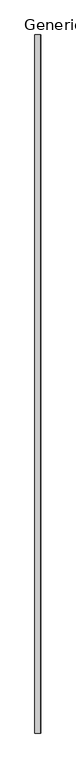
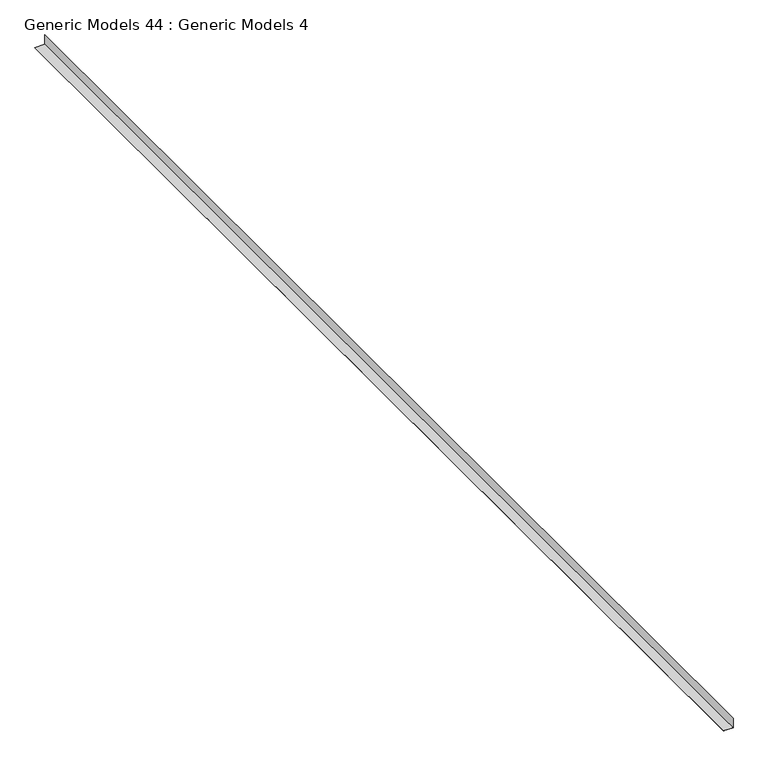
"""IFC4 building model written with IfcOpenShell, lengths in millimetres: proxy geometry, Generic Models 44 : Generic Models 4."""

from ifc_helpers import new_model, si_unit, frame, origin, place, context, project, spatial, polyline, outline, extrude, source, transform, mapped, element, save


def generic_models_44_generic_models_4_7e18a4ae(model_context):
    return source(origin(), model_context, "Body", "SweptSolid", [
        extrude(outline(polyline([(126902.6261365, 8392.8791721), (126899.4518253, 8240.5122343), (126898.6582475, 8240.5287672), (126901.8487507, 8393.6729221), (127055.0261365, 8393.6729221), (127055.0261365, 8392.8791721), (126902.6261365, 8392.8791721)])), frame((0.0, -6864.9230338, 0.0), z_axis=(0.0, 1.0, 0.0), x_axis=(0.0, 0.0, 1.0)), (0.0, 0.0, 1.0), 18643.6),
    ])


if __name__ == "__main__":
    model = new_model("IFC4")
    model_context = context("Model", 3, world=origin())
    ifc_project = project(units=[si_unit("LENGTHUNIT", "METRE", prefix="MILLI")], contexts=[model_context])
    site = spatial("IfcSite", under=ifc_project)
    building = spatial("IfcBuilding", under=site)
    placement = place(None, origin())
    generic_models_44_generic_models_4_shape = generic_models_44_generic_models_4_7e18a4ae(model_context)
    element("IfcBuildingElementProxy", 1, Name="Generic Models 44 : Generic Models 4", ObjectType="Generic Models 44 : Generic Models 4", at=placement, inside=building, context=model_context, shape_type="MappedRepresentation", body=[
        mapped(generic_models_44_generic_models_4_shape, transform((0.0, 0.0, 0.0), x_axis=(1.0, 0.0, 0.0), y_axis=(0.0, 1.0, 0.0), z_axis=(0.0, 0.0, 1.0))),
    ])
    save(model, "model.ifc")

# Revit data of these elements
# Element 1 (IfcBuildingElementProxy, "Generic Models 44 : Generic Models 4")
#   Materials on its faces: "_16 GA. COPPER \"L\" FLASHING - (6\" HORZ. LEG - 4\" VERT. LEG)"
# Materials
#   "_16 GA. COPPER \"L\" FLASHING - (6\" HORZ. LEG - 4\" VERT. LEG)": class "Generic", colour RGB 156 184 169, transparency 0, Cost = 0
